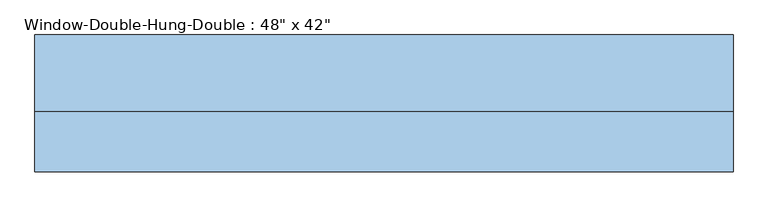
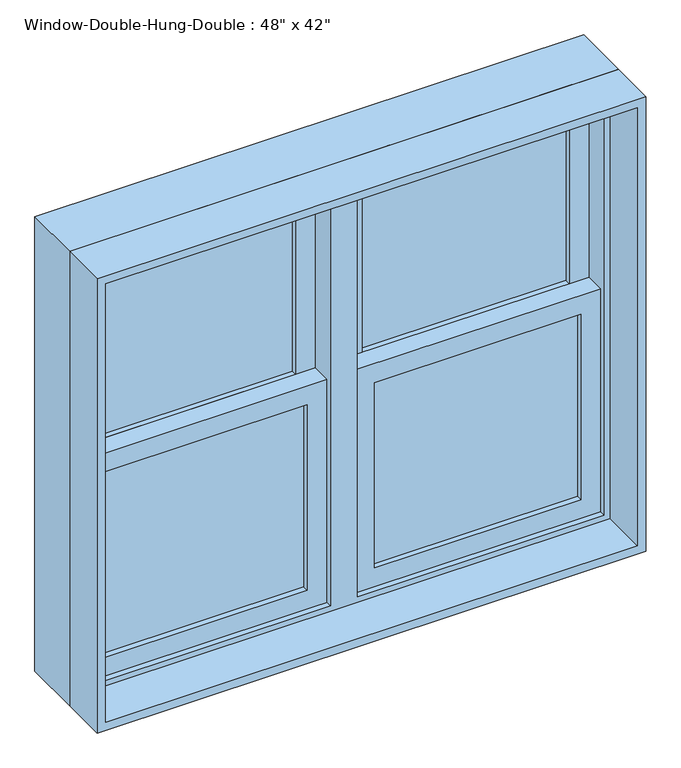
"""IFC4 building model written with IfcOpenShell, lengths in millimetres: window geometry."""

import ifcopenshell
import ifcopenshell.guid

model = None  # the IFC model being written
_history = None  # IfcOwnerHistory: only IFC2X3 demands one
_inside = {}  # id of a spatial element -> (the spatial element, [elements in it])
_under = {}  # id of a project, library or spatial element -> (it, [spatial elements below it])
_declared = {}  # id of a project -> (the project, [libraries it declares])
_typed = {}  # id of a type object -> (the type object, [elements of that type])
_made_of = {}  # id of a material, layer set ... -> (it, [elements and type objects made of it])


def new_model(schema):
    """Start an empty IFC model of exactly this schema.

    Asked for "IFC4X3", IfcOpenShell would pick the latest addendum, in which some entities
    have other attributes; the version numbers below select the first issue.
    IFC2X3 requires an IfcOwnerHistory on every rooted entity: one is made here for all.
    """
    global model, _history
    if schema == "IFC4X3":
        model = ifcopenshell.file(schema_version=(4, 3, 0, 0))
    else:
        model = ifcopenshell.file(schema=schema)
    _inside.clear()
    _under.clear()
    _declared.clear()
    _typed.clear()
    _made_of.clear()
    _history = None
    if model.schema == "IFC2X3":
        org = make("IfcOrganization", Name="unknown")
        user = make(
            "IfcPersonAndOrganization",
            ThePerson=make("IfcPerson", FamilyName="unknown"),
            TheOrganization=org,
        )
        app = make(
            "IfcApplication",
            ApplicationDeveloper=org,
            Version="unknown",
            ApplicationFullName="unknown",
            ApplicationIdentifier="unknown",
        )
        _history = make(
            "IfcOwnerHistory",
            OwningUser=user,
            OwningApplication=app,
            ChangeAction="ADDED",
            CreationDate=0,
        )
    return model


def make(cls, **values):
    """One entity of the class cls with the attributes given. An attribute that is None is left unset."""
    return model.create_entity(
        cls, **{name: value for name, value in values.items() if value is not None}
    )


def rooted(cls, **values):
    """An entity with a GlobalId (a new one), such as an element, a storey or a relation."""
    return make(cls, GlobalId=ifcopenshell.guid.new(), OwnerHistory=_history, **values)


def si_unit(unit_type, name, prefix=None):
    """IfcSIUnit, for example si_unit("LENGTHUNIT", "METRE", prefix="MILLI")."""
    return make("IfcSIUnit", UnitType=unit_type, Prefix=prefix, Name=name)


def assignment(units):
    """IfcUnitAssignment: the units of a project."""
    return None if units is None else make("IfcUnitAssignment", Units=units)


def point(xyz):
    """IfcCartesianPoint."""
    return None if xyz is None else make("IfcCartesianPoint", Coordinates=xyz)


def direction(xyz):
    """IfcDirection."""
    return None if xyz is None else make("IfcDirection", DirectionRatios=xyz)


def frame(location, z_axis=None, x_axis=None):
    """IfcAxis2Placement3D, a coordinate frame: its origin and axes. An axis left out is left unset."""
    return make(
        "IfcAxis2Placement3D",
        Location=point(location),
        Axis=direction(z_axis),
        RefDirection=direction(x_axis),
    )


def origin():
    """The frame at (0, 0, 0) with its axes left unset."""
    return frame((0.0, 0.0, 0.0))


def place(relative_to, where):
    """IfcLocalPlacement: puts the frame where relative to a parent placement (None: the world)."""
    return make(
        "IfcLocalPlacement", PlacementRelTo=relative_to, RelativePlacement=where
    )


def context(
    kind, dimensions, precision=None, world=None, true_north=None, identifier=None
):
    """IfcGeometricRepresentationContext, for example the 3D "Model" context."""
    return make(
        "IfcGeometricRepresentationContext",
        ContextIdentifier=identifier,
        ContextType=kind,
        CoordinateSpaceDimension=dimensions,
        Precision=precision,
        WorldCoordinateSystem=world,
        TrueNorth=true_north,
    )


def project(units=None, contexts=None):
    """IfcProject with its units and contexts."""
    return rooted(
        "IfcProject",
        Name="project",
        RepresentationContexts=contexts,
        UnitsInContext=assignment(units),
    )


def spatial(cls, under=None, at=None, **own):
    """A site, building, storey or space (cls), placed at a placement, below another one or the project."""
    s = rooted(cls, ObjectPlacement=at, **own)
    if under is not None:
        _under.setdefault(under.id(), (under, []))[1].append(s)
    return s


def polyline(points):
    """IfcPolyline through the points."""
    return make("IfcPolyline", Points=[point(p) for p in points])


def outline(outer, holes=None, kind="AREA"):
    """IfcArbitraryClosedProfileDef: a profile drawn as a closed curve; with holes, ...WithVoids."""
    if holes is None:
        return make("IfcArbitraryClosedProfileDef", ProfileType=kind, OuterCurve=outer)
    return make(
        "IfcArbitraryProfileDefWithVoids",
        ProfileType=kind,
        OuterCurve=outer,
        InnerCurves=holes,
    )


def extrude(swept, where, along, depth):
    """IfcExtrudedAreaSolid: the profile swept, set in the frame where, extruded along a direction by depth."""
    return make(
        "IfcExtrudedAreaSolid",
        SweptArea=swept,
        Position=where,
        ExtrudedDirection=direction(along),
        Depth=depth,
    )


def shape(context_of_items, identifier, shape_type, items):
    """IfcShapeRepresentation: the items that make up one representation, for example the "Body"."""
    return make(
        "IfcShapeRepresentation",
        ContextOfItems=context_of_items,
        RepresentationIdentifier=identifier,
        RepresentationType=shape_type,
        Items=items,
    )


def source(mapping_origin, context_of_items, identifier, shape_type, items):
    """IfcRepresentationMap: a shape defined once, which mapped items show again and again."""
    return make(
        "IfcRepresentationMap",
        MappingOrigin=mapping_origin,
        MappedRepresentation=shape(context_of_items, identifier, shape_type, items),
    )


def transform(
    local_origin,
    x_axis=None,
    y_axis=None,
    z_axis=None,
    scale=None,
    scale2=None,
    scale3=None,
    uniform=True,
):
    """IfcCartesianTransformationOperator3D, or its non-uniform kind. x_axis, y_axis, z_axis: its Axis1, 2, 3."""
    if uniform:
        return make(
            "IfcCartesianTransformationOperator3D",
            Axis1=direction(x_axis),
            Axis2=direction(y_axis),
            LocalOrigin=point(local_origin),
            Scale=scale,
            Axis3=direction(z_axis),
        )
    return make(
        "IfcCartesianTransformationOperator3DnonUniform",
        Axis1=direction(x_axis),
        Axis2=direction(y_axis),
        LocalOrigin=point(local_origin),
        Scale=scale,
        Axis3=direction(z_axis),
        Scale2=scale2,
        Scale3=scale3,
    )


def mapped(mapping_source, mapping_target):
    """IfcMappedItem: shows the shape of a source again, moved by a transform."""
    return make(
        "IfcMappedItem", MappingSource=mapping_source, MappingTarget=mapping_target
    )


def made_of(thing, what):
    """Note that an element or type object is made of a material, layer set ...; save() writes the relation."""
    if what is not None:
        _made_of.setdefault(what.id(), (what, []))[1].append(thing)
    return thing


def element(
    cls,
    number,
    at=None,
    inside=None,
    cuts=None,
    type_object=None,
    material=None,
    context=None,
    identifier="Body",
    shape_type=None,
    held_by="IfcProductDefinitionShape",
    body=None,
    shapes=None,
    **own,
):
    """One element of the class cls, such as IfcWall. Its Tag is "e" and its number.

    at: its placement. inside: the storey or other place that contains it. cuts: it is an
    opening in that element (IfcRelVoidsElement). A single representation is given by context,
    identifier, shape_type and body (its items); several are given by shapes. held_by: the class
    of the entity that holds the representations. save() writes the other relations.
    """
    e = rooted(cls, Tag="e%d" % number, ObjectPlacement=at, **own)
    if body is not None:
        shapes = [shape(context, identifier, shape_type, body)]
    if shapes is not None:
        e.Representation = make(held_by, Representations=shapes)
    if inside is not None:
        _inside.setdefault(inside.id(), (inside, []))[1].append(e)
    if cuts is not None:
        rooted(
            "IfcRelVoidsElement", RelatingBuildingElement=cuts, RelatedOpeningElement=e
        )
    if type_object is not None:
        _typed.setdefault(type_object.id(), (type_object, []))[1].append(e)
    return made_of(e, material)


def aggregate(whole, parts):
    """IfcRelAggregates: a whole, such as a stair, and the parts it consists of."""
    return rooted("IfcRelAggregates", RelatingObject=whole, RelatedObjects=parts)


def save(model, path):
    """Write the relations noted so far, then the file.

    IfcRelAggregates (storeys below a building ...), IfcRelContainedInSpatialStructure (elements
    in a storey), IfcRelDefinesByType, IfcRelAssociatesMaterial and IfcRelDeclares: one each for
    every whole, place, type object, material and project.
    """
    for whole, parts in _under.values():
        aggregate(whole, parts)
    for where, things in _inside.values():
        rooted(
            "IfcRelContainedInSpatialStructure",
            RelatedElements=things,
            RelatingStructure=where,
        )
    for kind, things in _typed.values():
        rooted("IfcRelDefinesByType", RelatedObjects=things, RelatingType=kind)
    for what, things in _made_of.values():
        rooted("IfcRelAssociatesMaterial", RelatedObjects=things, RelatingMaterial=what)
    for by, libraries in _declared.values():
        rooted("IfcRelDeclares", RelatingContext=by, RelatedDefinitions=libraries)
    model.write(path)


def window_9e3aa26a(model_context):
    return source(origin(), model_context, "Body", "SweptSolid", [
        extrude(outline(polyline([(1981.2, 609.6), (1981.2, -609.6), (914.4, -609.6), (914.4, 609.6), (1981.2, 609.6)]), holes=[polyline([(946.15, -577.85), (1949.45, -577.85), (1949.45, -30.1625), (946.15, -30.1625), (946.15, -577.85)]), polyline([(946.15, 577.85), (946.15, 30.1625), (1949.45, 30.1625), (1949.45, 577.85), (946.15, 577.85)])]), frame((0.0, -4.3, 0.0), z_axis=(0.0, 1.0, 0.0), x_axis=(0.0, 0.0, 1.0)), (0.0, 0.0, 1.0), 133.35),
        extrude(outline(polyline([(-533.4, 40.15), (-74.6125, 40.15), (-74.6125, 33.8), (-533.4, 33.8), (-533.4, 40.15)])), frame((0.0, 0.0, 990.6), z_axis=(0.0, 0.0, 1.0), x_axis=(1.0, 0.0, 0.0)), (0.0, 0.0, 1.0), 434.975),
        extrude(outline(polyline([(-74.6125, 27.45), (-74.6125, 21.1), (-533.4, 21.1), (-533.4, 27.45), (-74.6125, 27.45)])), frame((0.0, 0.0, 990.6), z_axis=(0.0, 0.0, 1.0), x_axis=(1.0, 0.0, 0.0)), (0.0, 0.0, 1.0), 434.975),
        extrude(outline(polyline([(-533.4, 84.6), (-74.6125, 84.6), (-74.6125, 78.25), (-533.4, 78.25), (-533.4, 84.6)])), frame((0.0, 0.0, 1470.025), z_axis=(0.0, 0.0, 1.0), x_axis=(1.0, 0.0, 0.0)), (0.0, 0.0, 1.0), 434.975),
        extrude(outline(polyline([(-74.6125, 71.9), (-74.6125, 65.55), (-533.4, 65.55), (-533.4, 71.9), (-74.6125, 71.9)])), frame((0.0, 0.0, 1470.025), z_axis=(0.0, 0.0, 1.0), x_axis=(1.0, 0.0, 0.0)), (0.0, 0.0, 1.0), 434.975),
        extrude(outline(polyline([(1470.025, -577.85), (946.15, -577.85), (946.15, -30.1625), (1470.025, -30.1625), (1470.025, -577.85)]), holes=[polyline([(1425.575, -74.6125), (990.6, -74.6125), (990.6, -533.4), (1425.575, -533.4), (1425.575, -74.6125)])]), frame((0.0, 8.4, 0.0), z_axis=(0.0, 1.0, 0.0), x_axis=(0.0, 0.0, 1.0)), (0.0, 0.0, 1.0), 44.45),
        extrude(outline(polyline([(1949.45, -577.85), (1425.575, -577.85), (1425.575, -30.1625), (1949.45, -30.1625), (1949.45, -577.85)]), holes=[polyline([(1905.0, -74.6125), (1470.025, -74.6125), (1470.025, -533.4), (1905.0, -533.4), (1905.0, -74.6125)])]), frame((0.0, 52.85, 0.0), z_axis=(0.0, 1.0, 0.0), x_axis=(0.0, 0.0, 1.0)), (0.0, 0.0, 1.0), 44.45),
        extrude(outline(polyline([(533.4, 40.15), (533.4, 33.8), (74.6125, 33.8), (74.6125, 40.15), (533.4, 40.15)])), frame((0.0, 0.0, 990.6), z_axis=(0.0, 0.0, 1.0), x_axis=(1.0, 0.0, 0.0)), (0.0, 0.0, 1.0), 434.975),
        extrude(outline(polyline([(74.6125, 27.45), (533.4, 27.45), (533.4, 21.1), (74.6125, 21.1), (74.6125, 27.45)])), frame((0.0, 0.0, 990.6), z_axis=(0.0, 0.0, 1.0), x_axis=(1.0, 0.0, 0.0)), (0.0, 0.0, 1.0), 434.975),
        extrude(outline(polyline([(533.4, 84.6), (533.4, 78.25), (74.6125, 78.25), (74.6125, 84.6), (533.4, 84.6)])), frame((0.0, 0.0, 1470.025), z_axis=(0.0, 0.0, 1.0), x_axis=(1.0, 0.0, 0.0)), (0.0, 0.0, 1.0), 434.975),
        extrude(outline(polyline([(74.6125, 71.9), (533.4, 71.9), (533.4, 65.55), (74.6125, 65.55), (74.6125, 71.9)])), frame((0.0, 0.0, 1470.025), z_axis=(0.0, 0.0, 1.0), x_axis=(1.0, 0.0, 0.0)), (0.0, 0.0, 1.0), 434.975),
        extrude(outline(polyline([(1470.025, 30.1625), (946.15, 30.1625), (946.15, 577.85), (1470.025, 577.85), (1470.025, 30.1625)]), holes=[polyline([(1425.575, 533.4), (990.6, 533.4), (990.6, 74.6125), (1425.575, 74.6125), (1425.575, 533.4)])]), frame((0.0, 8.4, 0.0), z_axis=(0.0, 1.0, 0.0), x_axis=(0.0, 0.0, 1.0)), (0.0, 0.0, 1.0), 44.45),
        extrude(outline(polyline([(1949.45, 30.1625), (1425.575, 30.1625), (1425.575, 577.85), (1949.45, 577.85), (1949.45, 30.1625)]), holes=[polyline([(1905.0, 533.4), (1470.025, 533.4), (1470.025, 74.6125), (1905.0, 74.6125), (1905.0, 533.4)])]), frame((0.0, 52.85, 0.0), z_axis=(0.0, 1.0, 0.0), x_axis=(0.0, 0.0, 1.0)), (0.0, 0.0, 1.0), 44.45),
        extrude(outline(polyline([(1981.2, 609.6), (1981.2, -609.6), (914.4, -609.6), (914.4, 609.6), (1981.2, 609.6)]), holes=[polyline([(1962.15, 590.55), (933.45, 590.55), (933.45, -590.55), (1962.15, -590.55), (1962.15, 590.55)])]), frame((0.0, -110.0, 0.0), z_axis=(0.0, 1.0, 0.0), x_axis=(0.0, 0.0, 1.0)), (0.0, 0.0, 1.0), 105.7),
    ])


if __name__ == "__main__":
    model = new_model("IFC4")
    model_context = context("Model", 3, world=origin())
    ifc_project = project(units=[si_unit("LENGTHUNIT", "METRE", prefix="MILLI")], contexts=[model_context])
    site = spatial("IfcSite", under=ifc_project)
    building = spatial("IfcBuilding", under=site)
    placement = place(None, origin())
    window_shape = window_9e3aa26a(model_context)
    element("IfcWindow", 1, ObjectType="Window-Double-Hung-Double : 48\" x 42\"", at=placement, inside=building, context=model_context, shape_type="MappedRepresentation", body=[
        mapped(window_shape, transform((0.0, 0.0, 0.0), x_axis=(1.0, 0.0, 0.0), y_axis=(0.0, 1.0, 0.0), z_axis=(0.0, 0.0, 1.0))),
    ])
    save(model, "model.ifc")

# Revit data of these elements
# Type "Window-Double-Hung-Double : 48\" x 42\""
#   Type Mark = "32"
#   Fire Rating = "0.5h"
#   Construction Type Id = "DG-DR"
#   Assembly Code = "B2020100"
#   Analytic Construction = "Double glazing - domestic"
#   Wall Thickness [instance default] = 15.24 cm
#   Window Inset [instance default] = 0 cm
#   Visual Light Transmittance = 0.81
#   Thermal Resistance (R) = 0.319569 (m²·K)/W
#   Solar Heat Gain Coefficient = 0.76
#   Muntin Width = 45.8787 cm
#   Muntin Height = 43.4975 cm
#   Interior Wall Closure [instance default] = 3.81 cm
#   Rough Width = 123.19 cm
#   Rough Height = 107.95 cm
#   Frame Extension [instance default] = 3.175 cm
#   Exterior Wall Closure [instance default] = 1.27 cm
#   Extension Jamb [instance default] = 3.81 cm
#   Heat Transfer Coefficient (U) = 3.12929 W/(m²·K)
#   Height = 106.68 cm
#   Width = 121.92 cm
#   Top Muntin Visibility = yes
#   Indicator Visibility [instance default] = yes
#   Extension Jamb Visibility [instance default] = yes
#   Interior Trim Visibility [instance default] = yes
#   Exterior Trim Visibility [instance default] = yes
#   Bottom Muntin Visibility = yes
#   Muntin Pattern = Muntin Pattern_2x2 : Muntin Pattern_2x2
#   Interior Trim Material = Wood - Stained
#   Interior Trim = Trim-Window-Interior-Flat : Picture Frame
#   Exterior Trim Material = Clad - White
#   Exterior Trim = Trim-Window-Exterior-Flat : with Sill
#   Glass Panel Material = Glass
#   Exterior Frame Material = Clad - White
#   Interior Frame Material = Wood - Stained
#   Wall Closure = (empty or 0)
# Element 1 (IfcWindow, "Window-Double-Hung-Double : 48\" x 42\"")
#   Wall Thickness = 22 cm
#   Extension Jamb = 10.57 cm
#   Materials on its faces: "Wood - Stained", "Glass", "Clad - White"
# Materials
#   "Wood - Stained": class "Wood", colour RGB 224 178 126, transparency 0, Cost = 0
#   "Clad - White": class "Wood", colour RGB 242 242 238, transparency 0, Cost = 0
#   "Glass": class "Glass", colour RGB 0 128 192, transparency 0.9, Description = "Soda Lime Glass", Cost = 0
